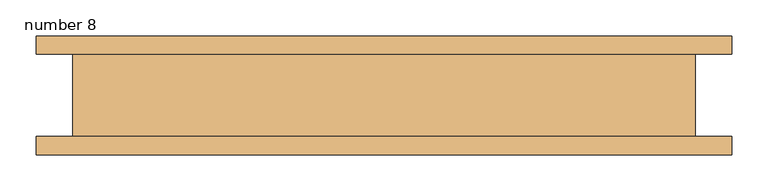
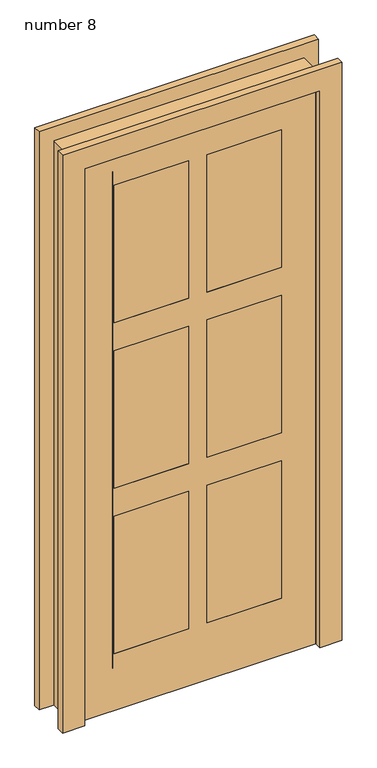
"""IFC4 building model written with IfcOpenShell, lengths in millimetres: door geometry, Doors-Supa_Doors-600_Glass : number 8."""

from ifc_helpers import new_model, si_unit, frame, origin, place, context, project, spatial, polyline, outline, extrude, source, transform, mapped, element, save


def number_8_34e83a0d(model_context):
    return source(origin(), model_context, "Body", "SweptSolid", [
        extrude(outline(polyline([(0.0, 431.8000001), (2057.4000001, 431.8000001), (2057.4000001, -431.8000001), (0.0, -431.8000001), (0.0, -406.4000001), (2032.0000001, -406.4000001), (2032.0000001, 406.4000001), (0.0, 406.4000001), (0.0, 431.8000001)])), frame((0.0, -57.15, 0.0), z_axis=(0.0, 1.0, 0.0), x_axis=(0.0, 0.0, 1.0)), (0.0, 0.0, 1.0), 114.3),
        extrude(outline(polyline([(0.0, 406.4000001), (2032.0000001, 406.4000001), (2032.0000001, -406.4000001), (0.0, -406.4000001), (0.0, 406.4000001)]), holes=[polyline([(206.375, 31.75), (708.025, 31.75), (708.025, 288.925), (206.375, 288.925), (206.375, 31.75)]), polyline([(1914.5250001, 31.75), (1914.5250001, 288.925), (1412.8750001, 288.925), (1412.8750001, 31.75), (1914.5250001, 31.75)]), polyline([(1412.8750001, -288.925), (1914.5250001, -288.925), (1914.5250001, -31.75), (1412.8750001, -31.75), (1412.8750001, -288.925)]), polyline([(1311.2750001, 31.75), (1311.2750001, 288.925), (809.625, 288.925), (809.625, 31.75), (1311.2750001, 31.75)]), polyline([(809.625, -288.925), (1311.2750001, -288.925), (1311.2750001, -31.75), (809.625, -31.75), (809.625, -288.925)]), polyline([(206.375, -288.925), (708.025, -288.925), (708.025, -31.75), (206.375, -31.75), (206.375, -288.925)])]), frame((0.0, -57.15, 0.0), z_axis=(0.0, 1.0, 0.0), x_axis=(0.0, 0.0, 1.0)), (0.0, 0.0, 1.0), 44.45),
        extrude(outline(polyline([(2032.0000001, -406.4000001), (2032.0000001, 406.4000001), (0.0, 406.4000001), (0.0, 482.6000001), (2108.2000001, 482.6000001), (2108.2000001, -482.6000001), (0.0, -482.6000001), (0.0, -406.4000001), (2032.0000001, -406.4000001)])), frame((0.0, 57.15, 0.0), z_axis=(0.0, 1.0, 0.0), x_axis=(0.0, 0.0, 1.0)), (0.0, 0.0, 1.0), 25.4),
        extrude(outline(polyline([(2032.0000001, -406.4000001), (2032.0000001, 406.4000001), (0.0, 406.4000001), (0.0, 482.6000001), (2108.2000001, 482.6000001), (2108.2000001, -482.6000001), (0.0, -482.6000001), (0.0, -406.4000001), (2032.0000001, -406.4000001)])), frame((0.0, -82.55, 0.0), z_axis=(0.0, 1.0, 0.0), x_axis=(0.0, 0.0, 1.0)), (0.0, 0.0, 1.0), 25.4),
        extrude(outline(polyline([(295.2750001, -57.15), (-295.2750001, -57.15), (-295.2750001, -50.8), (295.2750001, -50.8), (295.2750001, -57.15)])), frame((0.0, 0.0, 155.575), z_axis=(0.0, 0.0, 1.0), x_axis=(1.0, 0.0, 0.0)), (0.0, 0.0, 1.0), 1809.75),
    ])


if __name__ == "__main__":
    model = new_model("IFC4")
    model_context = context("Model", 3, world=origin())
    ifc_project = project(units=[si_unit("LENGTHUNIT", "METRE", prefix="MILLI")], contexts=[model_context])
    site = spatial("IfcSite", under=ifc_project)
    building = spatial("IfcBuilding", under=site)
    placement = place(None, origin())
    number_8_shape = number_8_34e83a0d(model_context)
    element("IfcDoor", 1, ObjectType="Doors-Supa_Doors-600_Glass : number 8", at=placement, inside=building, context=model_context, shape_type="MappedRepresentation", body=[
        mapped(number_8_shape, transform((0.0, 0.0, 0.0), x_axis=(1.0, 0.0, 0.0), y_axis=(0.0, 1.0, 0.0), z_axis=(0.0, 0.0, 1.0))),
    ])
    save(model, "model.ifc")

# Revit data of these elements
# Type "Doors-Supa_Doors-600_Glass : number 8"
#   Type Mark = "66"
#   Youtube clip = ""
#   Weight Net (Kg) = "0"
#   Uniclass 2.0 Description = ""
#   Uniclass 2.0 Code = ""
#   Uniclass 1.4 Description = ""
#   Uniclass 1.4 Code = ""
#   URL = "http://supadoor.com/"
#   UNSPSC Name = ""
#   UNSPSC Code = ""
#   Technical description = "http://www.supadoor.com/technical-specifications/3-part-spec.html"
#   Sticking Type = "T"
#   Region South America = "All"
#   Region Oceania = "All"
#   Region North America = "All"
#   Region Middle East = "All"
#   Region Europe = "All"
#   Region Asia = "All"
#   Region Antarctica = "All"
#   Region Africa = "All"
#   QR code = "http://supa-doors.bimobject.com/Glass_Doors_6-Panel"
#   Product group = "Glass Doors"
#   Product family = "Doors"
#   Product data url = "http://supa-doors.bimobject.com/Glass_Doors_6-Panel"
#   Product certification = "http://www.supadoor.com/index.html#"
#   Product SKU = "Glass_Doors_6-Panel"
#   Product Page URL = "http://supadoor.com/standard_doors/panel/general_design.html"
#   Product Name = "600"
#   Product Guid = "b7bd9161-500c-4f3b-9e1f-f23124606a15"
#   Product Documentation Link = "http://supadoor.com/standard_doors/panel/pdf/X-600.pdf"
#   Panel Type = "SC2"
#   Nominal width = "0.00"
#   Nominal height = "0.00"
#   NBS Reference Description = ""
#   NBS Reference Code = ""
#   Model = "600"
#   Material = ""
#   Manufacturer url = "http://supadoor.com/"
#   Manufacturer name = "Supa Doors"
#   Manufacturer country = "United States"
#   Manufacturer = "Supa Doors, Inc."
#   Installation instructions = ""
#   IFC Classification = ""
#   Edition number = "0"
#   EAN code = ""
#   Design country = "United States"
#   Description = "6 Panel Door"
#   Depth = "0.00"
#   Date of publishing = "2014-08-01"
#   COBIe Type Category = ""
#   BIMobject category = ""
#   Analytic Construction = "<None>"
#   Top Rail = 0' - 4 5/8"
#   Thickness = 0' - 1 3/4"
#   Stile Width = 0' - 4 5/8"
#   Rough Width = 2' - 10"
#   Rough Height = 6' - 9"
#   Panel Height = 1' - 7 3/4"
#   Mullion = 0' - 4"
#   Jamb Thickness = 0' - 1"
#   Inset = 0' - 0"
#   Frame Projection Ext. = 0' - 1"
#   Frame Projection Int. = 0' - 1"
#   Frame Width = 0' - 3"
#   Height = 6' - 8"
#   Width = 2' - 8"
#   Center Mullion = 0' - 2 1/2"
#   Bottom Rail = 0' - 8 1/8"
#   Sticking T = yes
#   Sticking S = no
#   Sticking R = no
#   Sticking O = no
#   Sticking E = no
#   Sticking B = no
#   Panel F1 = yes
#   Define Thermal Properties by = 1
#   Door Trim = Wood - Supa Doors - Painted White
#   Door Panel = Wood - Supa Doors - MDF - White
#   Door Glass = Door - Architrave
#   Function = (empty or 0)
#   Wall Closure = (empty or 0)
# Element 1 (IfcDoor, "Doors-Supa_Doors-600_Glass : number 8")
#   Materials on its faces: "Wood - Supa Doors - Painted White", "Wood - Supa Doors - MDF - White", "Door - Architrave"
# Materials
#   "Wood - Supa Doors - Painted White": class "Unassigned", colour RGB 255 255 255, transparency 0
#   "Wood - Supa Doors - MDF - White": class "Unassigned", colour RGB 255 255 255, transparency 0
#   "Door - Architrave": class "Wood", colour RGB 192 192 192, transparency 0, Keynote = "P20", Cost = 0
